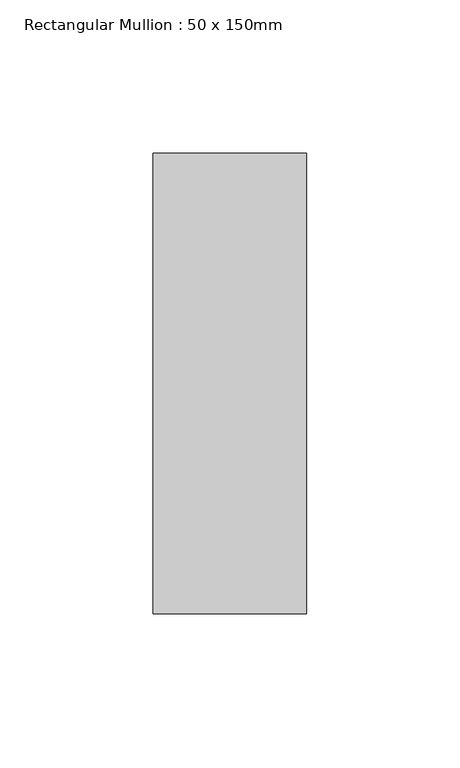
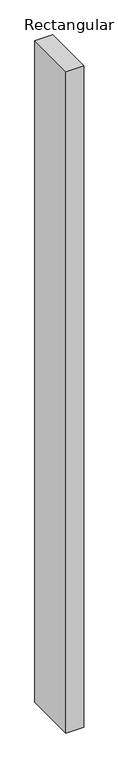
"""IFC4 building model written with IfcOpenShell, lengths in millimetres: member geometry, Rectangular Mullion : 50 x 150mm."""

from ifc_helpers import new_model, si_unit, frame, origin, place, context, project, spatial, polyline, outline, extrude, source, transform, mapped, element, save


def rectangular_mullion_50_x_150mm_825cde95(model_context):
    return source(origin(), model_context, "Body", "SweptSolid", [
        extrude(outline(polyline([(25.0, 75.0), (25.0, -75.0), (-25.0, -75.0), (-25.0, 75.0), (25.0, 75.0)])), frame((0.0, 0.0, -1948.3666666), z_axis=(0.0, 0.0, 1.0), x_axis=(1.0, 0.0, 0.0)), (0.0, 0.0, 1.0), 1948.3666666),
    ])


if __name__ == "__main__":
    model = new_model("IFC4")
    model_context = context("Model", 3, world=origin())
    ifc_project = project(units=[si_unit("LENGTHUNIT", "METRE", prefix="MILLI")], contexts=[model_context])
    site = spatial("IfcSite", under=ifc_project)
    building = spatial("IfcBuilding", under=site)
    placement = place(None, origin())
    rectangular_mullion_50_x_150mm_shape = rectangular_mullion_50_x_150mm_825cde95(model_context)
    element("IfcMember", 1, ObjectType="Rectangular Mullion : 50 x 150mm", at=placement, inside=building, context=model_context, shape_type="MappedRepresentation", body=[
        mapped(rectangular_mullion_50_x_150mm_shape, transform((0.0, 0.0, 0.0), x_axis=(1.0, 0.0, 0.0), y_axis=(0.0, 1.0, 0.0), z_axis=(0.0, 0.0, 1.0))),
    ])
    save(model, "model.ifc")

# Revit data of these elements
# Type "Rectangular Mullion : 50 x 150mm"
#   built-in parameter 1007304 = 0.492126 (stored number, unit not read)
#   built-in parameter 1007301 = 0.082021 (stored number, unit not read)
#   built-in parameter 1007300 = 0.082021 (stored number, unit not read)
# Element 1 (IfcMember, "Rectangular Mullion : 50 x 150mm")
#   Materials on its faces: "Metal - Aluminium"
# Materials
#   "Metal - Aluminium": class "Metal", colour RGB 247 247 247, transparency 0
